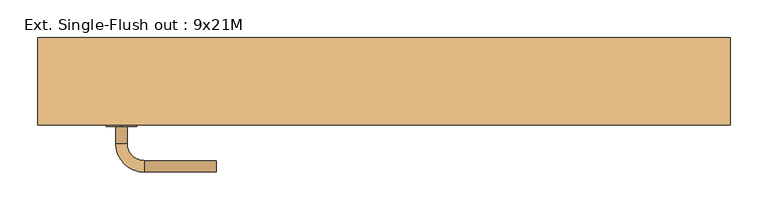
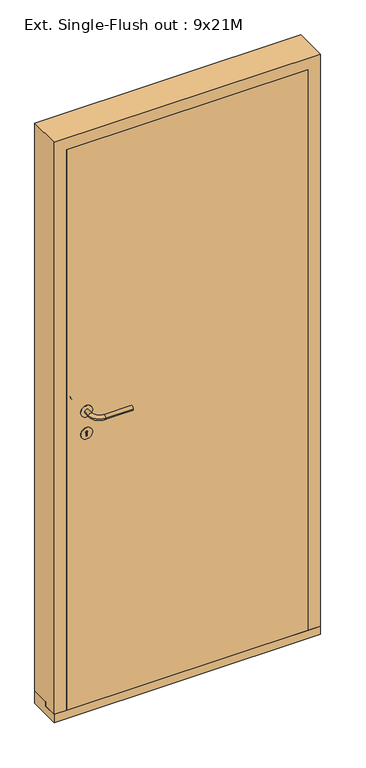
"""IFC4 building model written with IfcOpenShell, lengths in millimetres: door geometry, Ext. Single-Flush out : 9x21M."""

from ifc_helpers import new_model, si_unit, point, frame, frame_2d, origin, place, context, project, spatial, polyline, circle_curve, ellipse_curve, trimmed, segment, composite_curve, outline, extrude, faceted_brep, source, transform, mapped, element, save
from ifc_brep_helpers import plane_surface, cylinder_surface, revolved_surface, advanced_brep


def ext_single_flush_out_9x21m_b425c0d5(model_context):
    return source(origin(), model_context, "Body", "SolidModel", [
        extrude(outline(composite_curve([segment(trimmed(circle_curve(frame_2d((1090.0, -346.0)), 20.0), [point((1070.0, -346.0))], [point((1110.0, -346.0))], False, "CARTESIAN"), True, "CONTINUOUS"), segment(trimmed(circle_curve(frame_2d((1090.0, -346.0)), 20.0), [point((1110.0, -346.0))], [point((1070.0, -346.0))], False, "CARTESIAN"), True, "CONTINUOUS")], self_intersect=False)), frame((0.0, -186.0, 0.0), z_axis=(0.0, 1.0, 0.0), x_axis=(0.0, 0.0, 1.0)), (0.0, 0.0, 1.0), 2.0),
        advanced_brep(
        [(-353.5, -186.0, 1090.0), (-338.5, -186.0, 1090.0), (-338.5, -208.5, 1090.0), (-353.5, -208.5, 1090.0), (-316.0, -231.0, 1090.0), (-316.0, -246.0, 1090.0), (-221.0, -231.0, 1090.0), (-221.0, -246.0, 1090.0)],
        [
            (0, 1, circle_curve(frame((-346.0, -186.0, 1090.0), z_axis=(0.0, 1.0, 0.0), x_axis=(1.0, 0.0, 0.0)), 7.5)),
            (1, 0, circle_curve(frame((-346.0, -186.0, 1090.0), z_axis=(0.0, 1.0, 0.0), x_axis=(1.0, 0.0, 0.0)), 7.5)),
            (1, 2),
            (2, 3, circle_curve(frame((-346.0, -208.5, 1090.0), z_axis=(0.0, 1.0, 0.0), x_axis=(1.0, 0.0, 0.0)), 7.5)),
            (3, 0),
            (3, 2, circle_curve(frame((-346.0, -208.5, 1090.0), z_axis=(0.0, 1.0, 0.0), x_axis=(1.0, 0.0, 0.0)), 7.5)),
            (4, 5, circle_curve(frame((-316.0, -238.5, 1090.0), z_axis=(-1.0, 0.0, 0.0), x_axis=(0.0, 1.0, 0.0)), 7.5)),
            (5, 3, circle_curve(frame((-316.0, -208.5, 1090.0), z_axis=(0.0, 0.0, -1.0), x_axis=(-1.0, 0.0, 0.0)), 37.5)),
            (2, 4, circle_curve(frame((-316.0, -208.5, 1090.0), z_axis=(0.0, 0.0, 1.0), x_axis=(-1.0, 0.0, 0.0)), 22.5)),
            (5, 4, circle_curve(frame((-316.0, -238.5, 1090.0), z_axis=(-1.0, 0.0, 0.0), x_axis=(0.0, 1.0, 0.0)), 7.5)),
            (4, 6),
            (6, 7, circle_curve(frame((-221.0, -238.5, 1090.0), z_axis=(-1.0, 0.0, 0.0), x_axis=(0.0, 1.0, 0.0)), 7.5)),
            (7, 5),
            (7, 6, circle_curve(frame((-221.0, -238.5, 1090.0), z_axis=(-1.0, 0.0, 0.0), x_axis=(0.0, 1.0, 0.0)), 7.5)),
        ],
        [
            plane_surface(frame((-346.0, -186.0, 1090.0), z_axis=(0.0, 1.0, 0.0), x_axis=(0.0, 0.0, -1.0))),
            cylinder_surface(frame((-346.0, -186.0, 1090.0), z_axis=(0.0, 1.0, 0.0), x_axis=(1.0, 0.0, 0.0)), 7.5),
            revolved_surface(trimmed(ellipse_curve(frame((-346.0, -208.5, 1090.0), z_axis=(0.0, -1.0, 0.0), x_axis=(1.0, 0.0, 0.0)), 7.5, 7.5), [point((-353.5, -208.5, 1090.0))], [point((-338.5, -208.5, 1090.0))], True, "CARTESIAN"), (-316.0, -208.5, 1090.0), (0.0, 0.0, -1.0)),
            revolved_surface(trimmed(ellipse_curve(frame((-346.0, -208.5, 1090.0), z_axis=(0.0, -1.0, 0.0), x_axis=(1.0, 0.0, 0.0)), 7.5, 7.5), [point((-338.5, -208.5, 1090.0))], [point((-353.5, -208.5, 1090.0))], True, "CARTESIAN"), (-316.0, -208.5, 1090.0), (0.0, 0.0, -1.0)),
            cylinder_surface(frame((-316.0, -238.5, 1090.0), z_axis=(-1.0, 0.0, 0.0), x_axis=(0.0, 1.0, 0.0)), 7.5),
            plane_surface(frame((-221.0, -238.5, 1090.0), z_axis=(1.0, 0.0, 0.0), x_axis=(0.0, 0.0, -1.0))),
        ],
        [
            (0, [[1, 2]]),
            (1, [[3, 4, 5, -2]]),
            (1, [[-5, 6, -3, -1]]),
            (2, [[7, 8, -4, 9]]),
            (3, [[10, -9, -6, -8]]),
            (4, [[11, 12, 13, -7]]),
            (4, [[-13, 14, -11, -10]]),
            (5, [[-12, -14]]),
        ],
    ),
        extrude(outline(composite_curve([segment(trimmed(circle_curve(frame_2d((1010.0, -346.0)), 20.0), [point((990.0, -346.0))], [point((1030.0, -346.0))], False, "CARTESIAN"), True, "CONTINUOUS"), segment(trimmed(circle_curve(frame_2d((1010.0, -346.0)), 20.0), [point((1030.0, -346.0))], [point((990.0, -346.0))], False, "CARTESIAN"), True, "CONTINUOUS")], self_intersect=False), holes=[composite_curve([segment(trimmed(circle_curve(frame_2d((1015.0, -346.0)), 3.0), [point((1012.4019238, -347.5))], [point((1012.4019238, -344.5))], True, "CARTESIAN"), True, "CONTINUOUS"), segment(polyline([(1012.4019238, -344.5), (1000.0, -344.5), (1000.0, -347.5), (1012.4019238, -347.5)]), True, "CONTINUOUS")], self_intersect=False)]), frame((0.0, -186.0, 0.0), z_axis=(0.0, 1.0, 0.0), x_axis=(0.0, 0.0, 1.0)), (0.0, 0.0, 1.0), 2.0),
        extrude(outline(composite_curve([segment(trimmed(circle_curve(frame_2d((1090.0, -346.0)), 20.0), [point((1070.0, -346.0))], [point((1110.0, -346.0))], False, "CARTESIAN"), True, "CONTINUOUS"), segment(trimmed(circle_curve(frame_2d((1090.0, -346.0)), 20.0), [point((1110.0, -346.0))], [point((1070.0, -346.0))], False, "CARTESIAN"), True, "CONTINUOUS")], self_intersect=False)), frame((0.0, -134.0, 0.0), z_axis=(0.0, 1.0, 0.0), x_axis=(0.0, 0.0, 1.0)), (0.0, 0.0, 1.0), 2.0),
        advanced_brep(
        [(-353.5, -132.0, 1090.0), (-338.5, -132.0, 1090.0), (-353.5, -109.5, 1090.0), (-338.5, -109.5, 1090.0), (-316.0, -87.0, 1090.0), (-316.0, -72.0, 1090.0), (-221.0, -72.0, 1090.0), (-221.0, -87.0, 1090.0)],
        [
            (0, 1, circle_curve(frame((-346.0, -132.0, 1090.0), z_axis=(0.0, -1.0, 0.0), x_axis=(1.0, 0.0, 0.0)), 7.5)),
            (1, 0, circle_curve(frame((-346.0, -132.0, 1090.0), z_axis=(0.0, -1.0, 0.0), x_axis=(1.0, 0.0, 0.0)), 7.5)),
            (0, 2),
            (2, 3, circle_curve(frame((-346.0, -109.5, 1090.0), z_axis=(0.0, -1.0, 0.0), x_axis=(1.0, 0.0, 0.0)), 7.5)),
            (3, 1),
            (3, 2, circle_curve(frame((-346.0, -109.5, 1090.0), z_axis=(0.0, -1.0, 0.0), x_axis=(1.0, 0.0, 0.0)), 7.5)),
            (4, 3, circle_curve(frame((-316.0, -109.5, 1090.0), z_axis=(0.0, 0.0, 1.0), x_axis=(-1.0, 0.0, 0.0)), 22.5)),
            (2, 5, circle_curve(frame((-316.0, -109.5, 1090.0), z_axis=(0.0, 0.0, -1.0), x_axis=(-1.0, 0.0, 0.0)), 37.5)),
            (5, 4, circle_curve(frame((-316.0, -79.5, 1090.0), z_axis=(-1.0, 0.0, 0.0), x_axis=(0.0, -1.0, 0.0)), 7.5)),
            (4, 5, circle_curve(frame((-316.0, -79.5, 1090.0), z_axis=(-1.0, 0.0, 0.0), x_axis=(0.0, -1.0, 0.0)), 7.5)),
            (5, 6),
            (6, 7, circle_curve(frame((-221.0, -79.5, 1090.0), z_axis=(-1.0, 0.0, 0.0), x_axis=(0.0, -1.0, 0.0)), 7.5)),
            (7, 4),
            (7, 6, circle_curve(frame((-221.0, -79.5, 1090.0), z_axis=(-1.0, 0.0, 0.0), x_axis=(0.0, -1.0, 0.0)), 7.5)),
        ],
        [
            plane_surface(frame((-346.0, -132.0, 1090.0), z_axis=(0.0, -1.0, 0.0), x_axis=(0.0, 0.0, -1.0))),
            cylinder_surface(frame((-346.0, -132.0, 1090.0), z_axis=(0.0, -1.0, 0.0), x_axis=(1.0, 0.0, 0.0)), 7.5),
            revolved_surface(trimmed(ellipse_curve(frame((-346.0, -109.5, 1090.0), z_axis=(0.0, -1.0, 0.0), x_axis=(1.0, 0.0, 0.0)), 7.5, 7.5), [point((-353.5, -109.5, 1090.0))], [point((-338.5, -109.5, 1090.0))], True, "CARTESIAN"), (-316.0, -109.5, 1090.0), (0.0, 0.0, -1.0)),
            revolved_surface(trimmed(ellipse_curve(frame((-346.0, -109.5, 1090.0), z_axis=(0.0, -1.0, 0.0), x_axis=(1.0, 0.0, 0.0)), 7.5, 7.5), [point((-338.5, -109.5, 1090.0))], [point((-353.5, -109.5, 1090.0))], True, "CARTESIAN"), (-316.0, -109.5, 1090.0), (0.0, 0.0, -1.0)),
            cylinder_surface(frame((-316.0, -79.5, 1090.0), z_axis=(-1.0, 0.0, 0.0), x_axis=(0.0, -1.0, 0.0)), 7.5),
            plane_surface(frame((-221.0, -79.5, 1090.0), z_axis=(1.0, 0.0, 0.0), x_axis=(0.0, 0.0, -1.0))),
        ],
        [
            (0, [[1, 2]]),
            (1, [[-1, 3, 4, 5]]),
            (1, [[-2, -5, 6, -3]]),
            (2, [[7, -4, 8, 9]]),
            (3, [[-8, -6, -7, 10]]),
            (4, [[-9, 11, 12, 13]]),
            (4, [[-10, -13, 14, -11]]),
            (5, [[-14, -12]]),
        ],
    ),
        extrude(outline(composite_curve([segment(trimmed(circle_curve(frame_2d((1010.0, -346.0)), 20.0), [point((990.0, -346.0))], [point((1030.0, -346.0))], False, "CARTESIAN"), True, "CONTINUOUS"), segment(trimmed(circle_curve(frame_2d((1010.0, -346.0)), 20.0), [point((1030.0, -346.0))], [point((990.0, -346.0))], False, "CARTESIAN"), True, "CONTINUOUS")], self_intersect=False), holes=[composite_curve([segment(trimmed(circle_curve(frame_2d((1015.0, -346.0)), 3.0), [point((1012.4019238, -347.5))], [point((1012.4019238, -344.5))], True, "CARTESIAN"), True, "CONTINUOUS"), segment(polyline([(1012.4019238, -344.5), (1000.0, -344.5), (1000.0, -347.5), (1012.4019238, -347.5)]), True, "CONTINUOUS")], self_intersect=False)]), frame((0.0, -134.0, 0.0), z_axis=(0.0, 1.0, 0.0), x_axis=(0.0, 0.0, 1.0)), (0.0, 0.0, 1.0), 2.0),
        extrude(outline(polyline([(-414.0, -184.0), (-414.0, -134.0), (414.0, -134.0), (414.0, -184.0), (-414.0, -184.0)])), frame((0.0, 0.0, 30.0), z_axis=(0.0, 0.0, 1.0), x_axis=(1.0, 0.0, 0.0)), (0.0, 0.0, 1.0), 2028.0),
        faceted_brep([(414.0, -184.0, 2058.0), (414.0, -184.0, 30.0), (456.0, -184.0, 30.0), (456.0, -184.0, 2100.0), (-456.0, -184.0, 2100.0), (-456.0, -184.0, 30.0), (-414.0, -184.0, 30.0), (-414.0, -184.0, 2058.0), (-414.0, -134.0, 30.0), (-414.0, -134.0, 45.0), (-414.0, -134.0, 2058.0), (-456.0, -134.0, 30.0), (456.0, -134.0, 30.0), (414.0, -134.0, 30.0), (-456.0, -69.0, 2100.0), (-456.0, -69.0, 45.0), (-456.0, -134.0, 45.0), (456.0, -134.0, 45.0), (456.0, -69.0, 45.0), (456.0, -69.0, 2100.0), (414.0, -134.0, 2058.0), (414.0, -134.0, 45.0), (399.0, -69.0, 45.0), (399.0, -69.0, 2043.0), (-399.0, -69.0, 2043.0), (-399.0, -69.0, 45.0), (-399.0, -134.0, 45.0), (399.0, -134.0, 45.0), (-399.0, -134.0, 2043.0), (399.0, -134.0, 2043.0)], [[[0, 1, 2, 3, 4, 5, 6, 7]], [[7, 6, 8, 9, 10]], [[8, 6, 5, 11]], [[12, 2, 1, 13]], [[14, 15, 16, 11, 5, 4]], [[3, 2, 12, 17, 18, 19]], [[20, 21, 13, 1, 0]], [[19, 18, 22, 23, 24, 25, 15, 14]], [[16, 15, 25, 26, 9]], [[21, 27, 22, 18, 17]], [[9, 8, 11, 16]], [[17, 12, 13, 21]], [[28, 26, 25, 24]], [[23, 22, 27, 29]], [[29, 27, 21, 20, 10, 9, 26, 28]], [[3, 19, 14, 4]], [[23, 29, 28, 24]], [[7, 10, 20, 0]]]),
        extrude(outline(polyline([(-184.0, 30.0), (-134.0, 30.0), (-134.0, 45.0), (-69.0, 45.0), (-69.0, 0.0), (-184.0, 0.0), (-184.0, 30.0)])), frame((-456.0, 0.0, 0.0), z_axis=(1.0, 0.0, 0.0), x_axis=(0.0, 1.0, 0.0)), (0.0, 0.0, 1.0), 912.0),
    ])


if __name__ == "__main__":
    model = new_model("IFC4")
    model_context = context("Model", 3, world=origin())
    ifc_project = project(units=[si_unit("LENGTHUNIT", "METRE", prefix="MILLI")], contexts=[model_context])
    site = spatial("IfcSite", under=ifc_project)
    building = spatial("IfcBuilding", under=site)
    placement = place(None, origin())
    ext_single_flush_out_9x21m_shape = ext_single_flush_out_9x21m_b425c0d5(model_context)
    element("IfcDoor", 1, ObjectType="Ext. Single-Flush out : 9x21M", at=placement, inside=building, context=model_context, shape_type="MappedRepresentation", body=[
        mapped(ext_single_flush_out_9x21m_shape, transform((0.0, 0.0, 0.0), x_axis=(1.0, 0.0, 0.0), y_axis=(0.0, 1.0, 0.0), z_axis=(0.0, 0.0, 1.0))),
    ])
    save(model, "model.ifc")

# Revit data of these elements
# Type "Ext. Single-Flush out : 9x21M"
#   Type Mark = "63"
#   Sound Rating = ""
#   Opening Side [instance default] = "out"
#   Hinge Side [instance default] = ""
#   Creator Organization [instance default] = "© Danish Educational Content"
#   Creator Name [instance default] = "© Erik Falck Jørgensen"
#   Creator Build [instance default] = "2017.0301.0"
#   Analytic Construction = "<None>"
#   length#6 = -50 mm
#   length#4 = 120 mm
#   length#5 = 912 mm
#   length#3 = 30 mm
#   length#2 = 57 mm
#   length#1 = 0 mm
#   Thickness = 50 mm
#   Seal Width = 12 mm
#   Rough Width = 912 mm
#   Rough Height = 2100 mm
#   Rebate Depth = 50 mm
#   Rabbet Width = 15 mm
#   Rabbet Depth = 50 mm
#   Height = 2088 mm
#   Width = 888 mm
#   Handle From Side = 110 mm
#   Handle From Bottom = 1090 mm
#   Exterior Direction [instance default] = 0.00°
#   Case Depth = 115 mm
#   Case Width = 45 mm
#   Threshold = yes
#   Sealing = no
#   Hinging = yes
#   Wall Closure = 1
#   Function = 1
#   Panel = none
#   Handle Finish = none
#   Handle = element 632149
#   Case/Transom = none
#   Assembly Code = ""
# Element 1 (IfcDoor, "Ext. Single-Flush out : 9x21M")
#   Materials on its faces: "Stainless Steel, Polished", "Default Frame/Mullion (Interior/Exterior)", "Default Door Panel (Exterior/Interior)"
# Materials
#   "Stainless Steel, Polished": class "Metal", colour RGB 180 180 180, transparency 0, Description = "Rustfri stål, poleret", Cost = 0
#   "Default Frame/Mullion (Interior/Exterior)": class "Generic", colour RGB 205 205 205, transparency 0, Description = "Udefineret karm/ramme materiale", Cost = 0
#   "Default Door Panel (Exterior/Interior)": class "Generic", colour RGB 205 205 205, transparency 0, Description = "Udefineret dørplade materiale", Cost = 0
